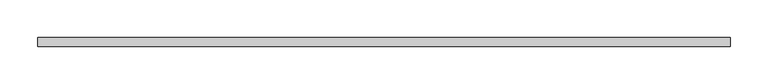
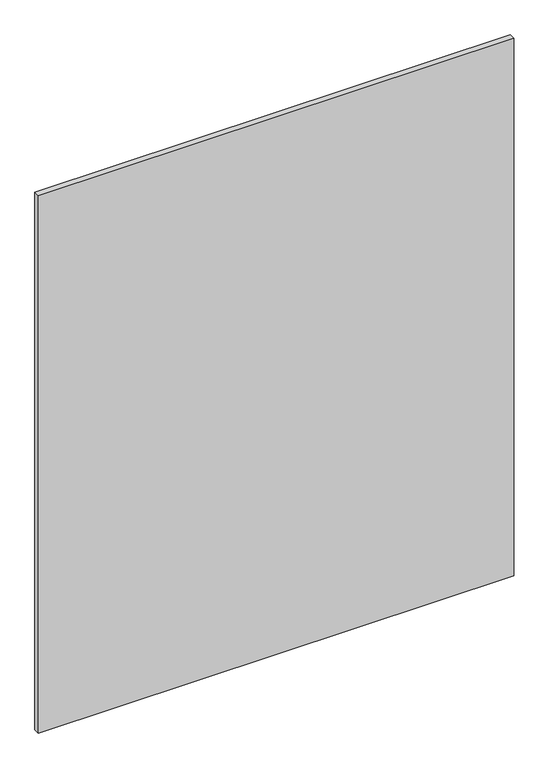
"""IFC4 building model written with IfcOpenShell, lengths in millimetres: railing geometry, ML_Painéis4 : ML_Painéis."""

from ifc_helpers import new_model, si_unit, frame, origin, place, context, project, spatial, polyline, outline, extrude, source, transform, mapped, element, save


def railing_29f9e2f6(model_context):
    return source(origin(), model_context, "Body", "SweptSolid", [
        extrude(outline(polyline([(-4674.5702584, 2133.3602771), (-4674.5702584, 2121.3602771), (-5595.5702584, 2121.3602771), (-5595.5702584, 2133.3602771), (-4674.5702584, 2133.3602771)])), frame((0.0, 0.0, 4122.0679199), z_axis=(0.0, 0.0, 1.0), x_axis=(1.0, 0.0, 0.0)), (0.0, 0.0, 1.0), 1100.0),
    ])


if __name__ == "__main__":
    model = new_model("IFC4")
    model_context = context("Model", 3, world=origin())
    ifc_project = project(units=[si_unit("LENGTHUNIT", "METRE", prefix="MILLI")], contexts=[model_context])
    site = spatial("IfcSite", under=ifc_project)
    building = spatial("IfcBuilding", under=site)
    placement = place(None, origin())
    railing_shape = railing_29f9e2f6(model_context)
    element("IfcRailing", 1, ObjectType="ML_Painéis4 : ML_Painéis", at=placement, inside=building, context=model_context, shape_type="MappedRepresentation", body=[
        mapped(railing_shape, transform((0.0, 0.0, 0.0), x_axis=(1.0, 0.0, 0.0), y_axis=(0.0, 1.0, 0.0), z_axis=(0.0, 0.0, 1.0))),
    ])
    save(model, "model.ifc")

# Revit data of these elements
# Type "ML_Painéis4 : ML_Painéis"
#   ME_Área [instance default] = 1.0131 m²
#   ME_Espessura [instance default] = 0.012 m
#   ME_Dist Painéis [instance default] = 0.002 m
#   ME_Compr Painéis [instance default] = 0.921 m
#   ME_Compr [instance default] = 0.925 m
#   ME_Altura [instance default] = 1.10 m
#   ME_Quant Painéis [instance default] = 3
#   ME_Painel Único [instance default] = yes
#   ME_Paineis Vários [instance default] = no
#   ME_Material Tipo Vidro [instance default] = .VIDRO GENÉRICO
# Element 1 (IfcRailing, "ML_Painéis4 : ML_Painéis")
#   Materials on its faces: ".VIDRO GENÉRICO"
# Materials
#   ".VIDRO GENÉRICO": class ".CC_VIDRO", colour RGB 0 128 192, transparency 0.9, Description = "Vidro comum", Cost = 0
